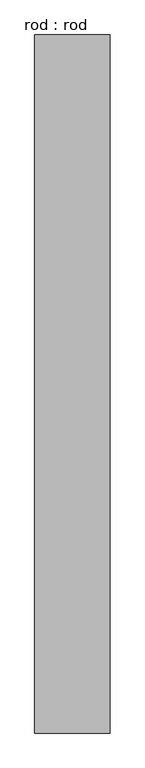
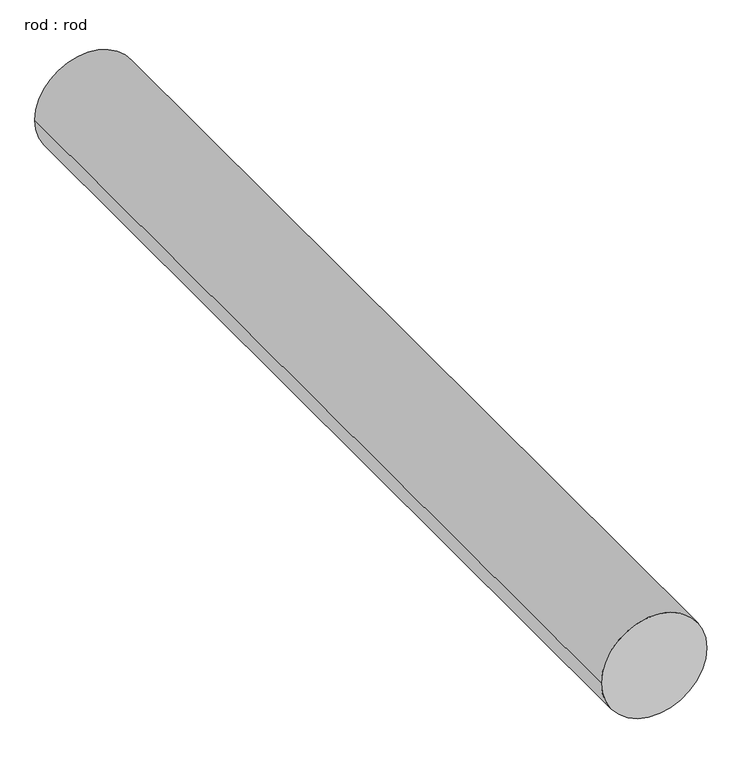
"""IFC4 building model written with IfcOpenShell, lengths in millimetres: proxy geometry, rod : rod."""

from ifc_helpers import new_model, si_unit, point, frame, frame_2d, origin, place, context, project, spatial, circle_curve, trimmed, segment, composite_curve, outline, extrude, source, transform, mapped, element, save


def rod_rod_81b04c94(model_context):
    return source(origin(), model_context, "Body", "SweptSolid", [
        extrude(outline(composite_curve([segment(trimmed(circle_curve(frame_2d((0.0108462, 0.0)), 200.0), [point((0.0108462, 200.0))], [point((0.0108462, -200.0))], False, "CARTESIAN"), True, "CONTINUOUS"), segment(trimmed(circle_curve(frame_2d((0.0108462, 0.0)), 200.0), [point((0.0108462, -200.0))], [point((0.0108462, 200.0))], False, "CARTESIAN"), True, "CONTINUOUS")], self_intersect=False)), frame((0.0, 2239.2032581, 0.0), z_axis=(0.0, 1.0, 0.0), x_axis=(0.0, 0.0, 1.0)), (0.0, 0.0, 1.0), 3707.0507145),
    ])


if __name__ == "__main__":
    model = new_model("IFC4")
    model_context = context("Model", 3, world=origin())
    ifc_project = project(units=[si_unit("LENGTHUNIT", "METRE", prefix="MILLI")], contexts=[model_context])
    site = spatial("IfcSite", under=ifc_project)
    building = spatial("IfcBuilding", under=site)
    placement = place(None, origin())
    rod_rod_shape = rod_rod_81b04c94(model_context)
    element("IfcBuildingElementProxy", 1, Name="rod : rod", ObjectType="rod : rod", at=placement, inside=building, context=model_context, shape_type="MappedRepresentation", body=[
        mapped(rod_rod_shape, transform((0.0, 0.0, 0.0), x_axis=(1.0, 0.0, 0.0), y_axis=(0.0, 1.0, 0.0), z_axis=(0.0, 0.0, 1.0))),
    ])
    save(model, "model.ifc")

# Revit data of these elements
# Type "rod : rod"
#   Default Elevation = 0
